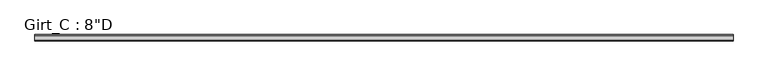
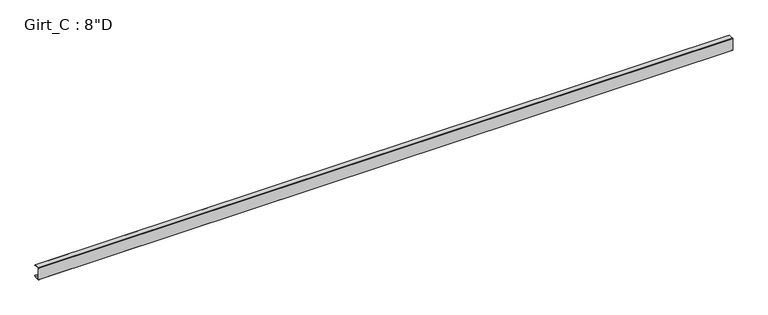
"""IFC4 building model written with IfcOpenShell, lengths in millimetres: beam geometry."""

from ifc_helpers import new_model, si_unit, point, frame, frame_2d, origin, place, context, project, spatial, polyline, circle_curve, trimmed, segment, composite_curve, outline, extrude, source, transform, mapped, element, save


def beam_b678a68b(model_context):
    return source(origin(), model_context, "Body", "SweptSolid", [
        extrude(outline(composite_curve([segment(polyline([(87.5109375, 101.6), (99.7560415, 87.0068534), (97.6278742, 85.221109), (86.2154765, 98.821875), (3.3005807, 98.821875)]), True, "CONTINUOUS"), segment(trimmed(circle_curve(frame_2d((3.3741066, 96.8381931)), 1.9850441), [point((3.3005807, 98.821875))], [point((1.3890625, 96.8381931))], True, "CARTESIAN"), True, "CONTINUOUS"), segment(polyline([(1.3890625, 96.8381931), (1.3890625, -96.8389339)]), True, "CONTINUOUS"), segment(trimmed(circle_curve(frame_2d((3.3748024, -96.8389339)), 1.9857399), [point((1.3890625, -96.8389339))], [point((3.2694106, -98.821875))], True, "CARTESIAN"), True, "CONTINUOUS"), segment(polyline([(3.2694106, -98.821875), (86.2154765, -98.821875), (97.6510975, -85.1934327), (99.7792647, -86.979177), (87.5109375, -101.6), (3.3734375, -101.6)]), True, "CONTINUOUS"), segment(trimmed(circle_curve(frame_2d((3.3734375, -96.8375)), 4.7625), [point((3.3734375, -101.6))], [point((-1.3890625, -96.8375))], False, "CARTESIAN"), True, "CONTINUOUS"), segment(polyline([(-1.3890625, -96.8375), (-1.3890625, 96.8375)]), True, "CONTINUOUS"), segment(trimmed(circle_curve(frame_2d((3.3734375, 96.8375)), 4.7625), [point((-1.3890625, 96.8375))], [point((3.3734375, 101.6))], False, "CARTESIAN"), True, "CONTINUOUS"), segment(polyline([(3.3734375, 101.6), (87.5109375, 101.6)]), True, "CONTINUOUS")], self_intersect=False)), frame((-5654.675, 0.0, 0.0), z_axis=(1.0, 0.0, 0.0), x_axis=(0.0, 1.0, 0.0)), (0.0, 0.0, 1.0), 11309.35),
    ])


if __name__ == "__main__":
    model = new_model("IFC4")
    model_context = context("Model", 3, world=origin())
    ifc_project = project(units=[si_unit("LENGTHUNIT", "METRE", prefix="MILLI")], contexts=[model_context])
    site = spatial("IfcSite", under=ifc_project)
    building = spatial("IfcBuilding", under=site)
    placement = place(None, origin())
    beam_shape = beam_b678a68b(model_context)
    element("IfcBeam", 1, ObjectType="Girt_C : 8\"D", at=placement, inside=building, context=model_context, shape_type="MappedRepresentation", body=[
        mapped(beam_shape, transform((0.0, 0.0, 0.0), x_axis=(1.0, 0.0, 0.0), y_axis=(0.0, 1.0, 0.0), z_axis=(0.0, 0.0, 1.0))),
    ])
    save(model, "model.ifc")

# Revit data of these elements
# Type "Girt_C : 8\"D"
#   half leg = 0' - 1 3/4"
#   Web_Thickness = 0' - 0 7/64"
#   Length [instance default] = 10' - 0"
#   Leg_1 = 0' - 3 1/2"
#   Height = 0' - 8"
#   Structural Material [instance default] = none
# Element 1 (IfcBeam, "Girt_C : 8\"D")
#   Structural Material = GALVANIZED 'CEE' SECTION (8.0x3.5C - SEE STRUCT. DWGS)
#   Materials on its faces: "GALVANIZED 'CEE' SECTION (8.0x3.5C - SEE STRUCT. DWGS)"
# Materials
#   "GALVANIZED 'CEE' SECTION (8.0x3.5C - SEE STRUCT. DWGS)": class "Metal", colour RGB 137 146 153, transparency 0, Description = "Steel, mill finish", Cost = 0
